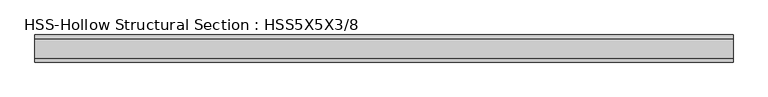
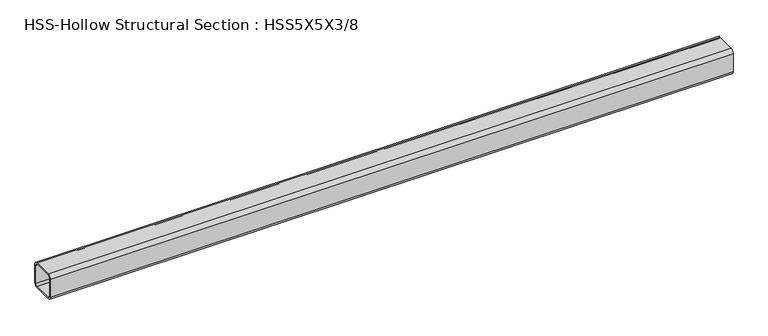
"""IFC4 building model written with IfcOpenShell, lengths in millimetres: member geometry, HSS-Hollow Structural Section : HSS5X5X3/8."""

from ifc_helpers import new_model, si_unit, point, frame, frame_2d, origin, place, context, project, spatial, polyline, circle_curve, trimmed, segment, composite_curve, outline, extrude, source, transform, mapped, element, save


def hss_hollow_structural_section_hss5x5x3_8_63cb5fcc(model_context):
    return source(origin(), model_context, "Body", "SweptSolid", [
        extrude(outline(composite_curve([segment(polyline([(63.5, 45.7708), (63.5, -45.7708)]), True, "CONTINUOUS"), segment(trimmed(circle_curve(frame_2d((45.7708, -45.7708)), 17.7292), [point((63.5, -45.7708))], [point((45.7708, -63.5))], False, "CARTESIAN"), True, "CONTINUOUS"), segment(polyline([(45.7708, -63.5), (-45.7708, -63.5)]), True, "CONTINUOUS"), segment(trimmed(circle_curve(frame_2d((-45.7708, -45.7708)), 17.7292), [point((-45.7708, -63.5))], [point((-63.5, -45.7708))], False, "CARTESIAN"), True, "CONTINUOUS"), segment(polyline([(-63.5, -45.7708), (-63.5, 45.7708)]), True, "CONTINUOUS"), segment(trimmed(circle_curve(frame_2d((-45.7708, 45.7708)), 17.7292), [point((-63.5, 45.7708))], [point((-45.7708, 63.5))], False, "CARTESIAN"), True, "CONTINUOUS"), segment(polyline([(-45.7708, 63.5), (45.7708, 63.5)]), True, "CONTINUOUS"), segment(trimmed(circle_curve(frame_2d((45.7708, 45.7708)), 17.7292), [point((45.7708, 63.5))], [point((63.5, 45.7708))], False, "CARTESIAN"), True, "CONTINUOUS")], self_intersect=False), holes=[composite_curve([segment(trimmed(circle_curve(frame_2d((-45.7708, 45.7708)), 8.8646), [point((-45.7708, 54.6354))], [point((-54.6354, 45.7708))], True, "CARTESIAN"), True, "CONTINUOUS"), segment(polyline([(-54.6354, 45.7708), (-54.6354, -45.7708)]), True, "CONTINUOUS"), segment(trimmed(circle_curve(frame_2d((-45.7708, -45.7708)), 8.8646), [point((-54.6354, -45.7708))], [point((-45.7708, -54.6354))], True, "CARTESIAN"), True, "CONTINUOUS"), segment(polyline([(-45.7708, -54.6354), (45.7708, -54.6354)]), True, "CONTINUOUS"), segment(trimmed(circle_curve(frame_2d((45.7708, -45.7708)), 8.8646), [point((45.7708, -54.6354))], [point((54.6354, -45.7708))], True, "CARTESIAN"), True, "CONTINUOUS"), segment(polyline([(54.6354, -45.7708), (54.6354, 45.7708)]), True, "CONTINUOUS"), segment(trimmed(circle_curve(frame_2d((45.7708, 45.7708)), 8.8646), [point((54.6354, 45.7708))], [point((45.7708, 54.6354))], True, "CARTESIAN"), True, "CONTINUOUS"), segment(polyline([(45.7708, 54.6354), (-45.7708, 54.6354)]), True, "CONTINUOUS")], self_intersect=False)]), frame((-1532.8473346, 0.0, 0.0), z_axis=(1.0, 0.0, 0.0), x_axis=(0.0, 1.0, 0.0)), (0.0, 0.0, 1.0), 3269.1115043),
    ])


if __name__ == "__main__":
    model = new_model("IFC4")
    model_context = context("Model", 3, world=origin())
    ifc_project = project(units=[si_unit("LENGTHUNIT", "METRE", prefix="MILLI")], contexts=[model_context])
    site = spatial("IfcSite", under=ifc_project)
    building = spatial("IfcBuilding", under=site)
    placement = place(None, origin())
    hss_hollow_structural_section_hss5x5x3_8_shape = hss_hollow_structural_section_hss5x5x3_8_63cb5fcc(model_context)
    element("IfcMember", 1, ObjectType="HSS-Hollow Structural Section : HSS5X5X3/8", at=placement, inside=building, context=model_context, shape_type="MappedRepresentation", body=[
        mapped(hss_hollow_structural_section_hss5x5x3_8_shape, transform((0.0, 0.0, 0.0), x_axis=(1.0, 0.0, 0.0), y_axis=(0.0, 1.0, 0.0), z_axis=(0.0, 0.0, 1.0))),
    ])
    save(model, "model.ifc")

# Revit data of these elements
# Type "HSS-Hollow Structural Section : HSS5X5X3/8"
#   Assembly Code = "B10"
#   Shape = "Square"
#   W = 22.3
#   Ht = 0' - 5"
#   Length [instance default] = 5' - 0"
#   b = 0' - 5"
#   kr = 0' - 0.698"
#   t = 0' - 0.349"
#   A = 0.0429167 SF
#   Structural Material [instance default] = Steel ASTM A500, Grade B, Rectangular and Square
# Element 1 (IfcMember, "HSS-Hollow Structural Section : HSS5X5X3/8")
#   Materials on its faces: "Steel ASTM A500, Grade B, Rectangular and Square"
# Materials
#   "Steel ASTM A500, Grade B, Rectangular and Square": class "Metal", colour RGB 199 199 199, transparency 0, Description = "Carbon steel", Cost = 0
